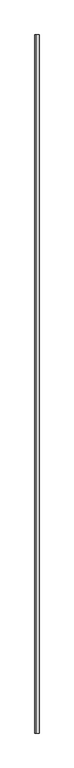
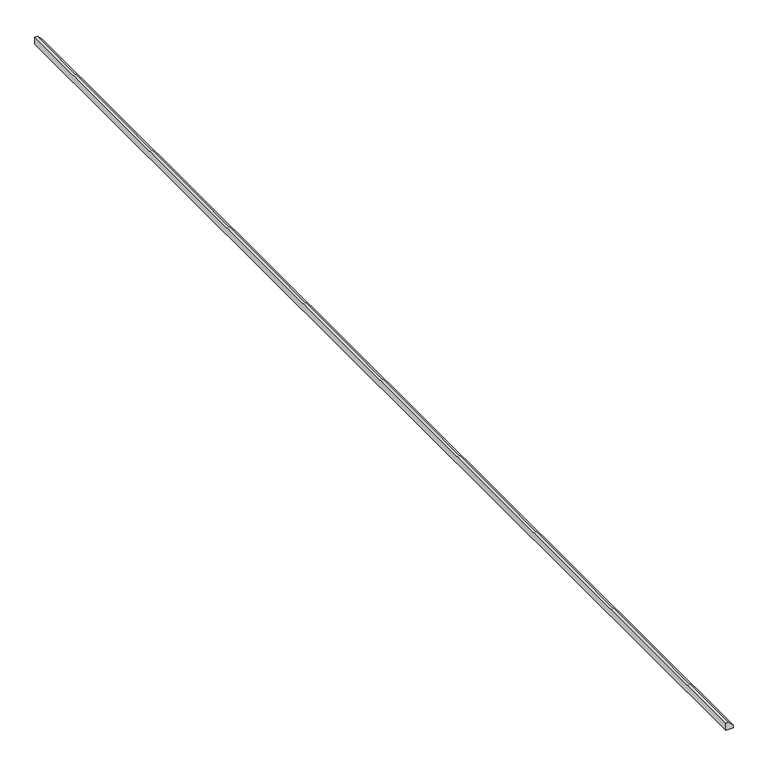
"""IFC4 building model written with IfcOpenShell, lengths in millimetres: proxy geometry, Stephan Brady5 : Stephan Brady."""

from ifc_helpers import new_model, si_unit, frame, origin, place, context, project, spatial, polyline, outline, extrude, source, transform, mapped, element, save


def generic_models_c530f3c3(model_context):
    return source(origin(), model_context, "Body", "SweptSolid", [
        extrude(outline(polyline([(3226.308, -9293.5068771), (3207.258, -9293.5068771), (3207.258, -9274.4568771), (3213.608, -9274.4568771), (3226.308, -9287.1568771), (3226.308, -9293.5068771)])), frame((0.0, -3268.5019926, 0.0), z_axis=(0.0, 1.0, 0.0), x_axis=(0.0, 0.0, 1.0)), (0.0, 0.0, 1.0), 3181.0024618),
    ])


if __name__ == "__main__":
    model = new_model("IFC4")
    model_context = context("Model", 3, world=origin())
    ifc_project = project(units=[si_unit("LENGTHUNIT", "METRE", prefix="MILLI")], contexts=[model_context])
    site = spatial("IfcSite", under=ifc_project)
    building = spatial("IfcBuilding", under=site)
    placement = place(None, origin())
    generic_models_shape = generic_models_c530f3c3(model_context)
    element("IfcBuildingElementProxy", 1, Name="Stephan Brady5 : Stephan Brady", ObjectType="Stephan Brady5 : Stephan Brady", at=placement, inside=building, context=model_context, shape_type="MappedRepresentation", body=[
        mapped(generic_models_shape, transform((0.0, 0.0, 0.0), x_axis=(1.0, 0.0, 0.0), y_axis=(0.0, 1.0, 0.0), z_axis=(0.0, 0.0, 1.0))),
    ])
    save(model, "model.ifc")

# Revit data of these elements
# Element 1 (IfcBuildingElementProxy, "Stephan Brady5 : Stephan Brady")
#   Materials on its faces: "Aluminum"
# Materials
#   "Aluminum": class "Metal", colour RGB 247 247 247, transparency 0, Description = "Aluminum 6061", Cost = 0
